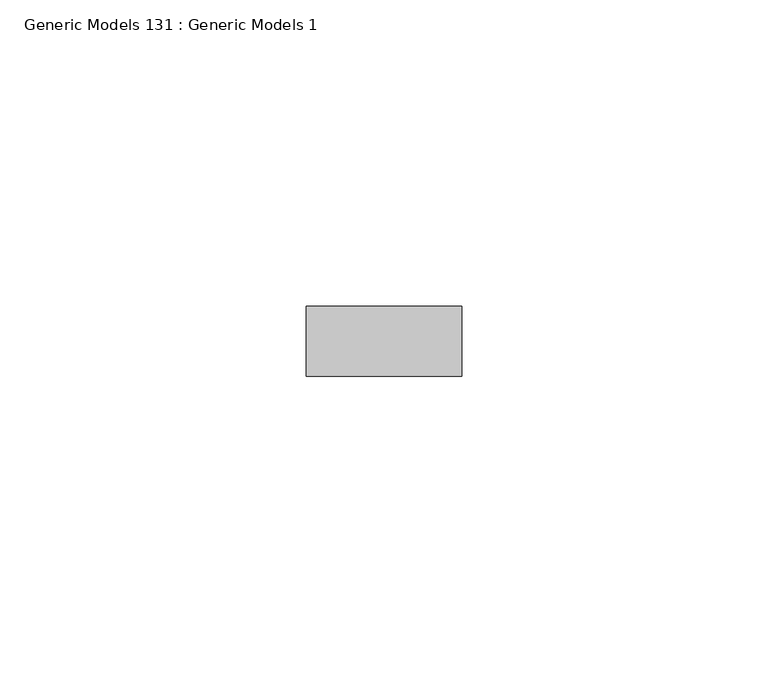
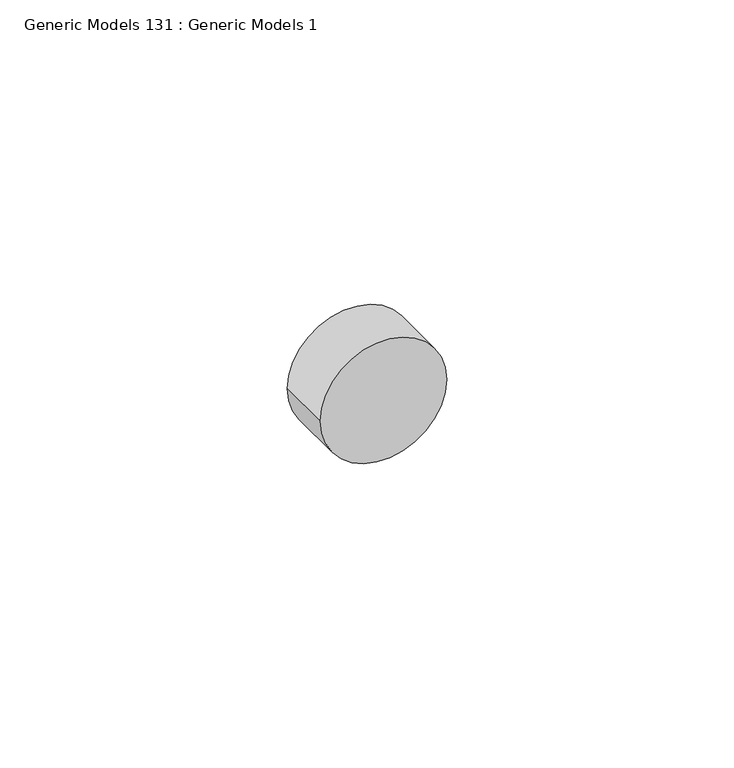
"""IFC4 building model written with IfcOpenShell, lengths in millimetres: proxy geometry, Generic Models 131 : Generic Models 1."""

from ifc_helpers import new_model, si_unit, point, frame, frame_2d, origin, place, context, project, spatial, circle_curve, trimmed, segment, composite_curve, outline, extrude, source, transform, mapped, element, save


def generic_models_131_generic_models_1_6fcba7fc(model_context):
    return source(origin(), model_context, "Body", "SweptSolid", [
        extrude(outline(composite_curve([segment(trimmed(circle_curve(frame_2d((38546.4677238, 7856.3346014)), 12.7), [point((38546.4677238, 7869.0346014))], [point((38546.4677238, 7843.6346014))], False, "CARTESIAN"), True, "CONTINUOUS"), segment(trimmed(circle_curve(frame_2d((38546.4677238, 7856.3346014)), 12.7), [point((38546.4677238, 7843.6346014))], [point((38546.4677238, 7869.0346014))], False, "CARTESIAN"), True, "CONTINUOUS")], self_intersect=False)), frame((0.0, 1836.9202358, 0.0), z_axis=(0.0, 1.0, 0.0), x_axis=(0.0, 0.0, 1.0)), (0.0, 0.0, 1.0), 11.4464372),
    ])


if __name__ == "__main__":
    model = new_model("IFC4")
    model_context = context("Model", 3, world=origin())
    ifc_project = project(units=[si_unit("LENGTHUNIT", "METRE", prefix="MILLI")], contexts=[model_context])
    site = spatial("IfcSite", under=ifc_project)
    building = spatial("IfcBuilding", under=site)
    placement = place(None, origin())
    generic_models_131_generic_models_1_shape = generic_models_131_generic_models_1_6fcba7fc(model_context)
    element("IfcBuildingElementProxy", 1, Name="Generic Models 131 : Generic Models 1", ObjectType="Generic Models 131 : Generic Models 1", at=placement, inside=building, context=model_context, shape_type="MappedRepresentation", body=[
        mapped(generic_models_131_generic_models_1_shape, transform((0.0, 0.0, 0.0), x_axis=(1.0, 0.0, 0.0), y_axis=(0.0, 1.0, 0.0), z_axis=(0.0, 0.0, 1.0))),
    ])
    save(model, "model.ifc")

# Revit data of these elements
# Element 1 (IfcBuildingElementProxy, "Generic Models 131 : Generic Models 1")
#   Materials on its faces: "S.S. LAG BOLT - SEE STRUCT. DWGS"
# Materials
#   "S.S. LAG BOLT - SEE STRUCT. DWGS": class "Generic", colour RGB 120 120 120, transparency 0, Cost = 0
